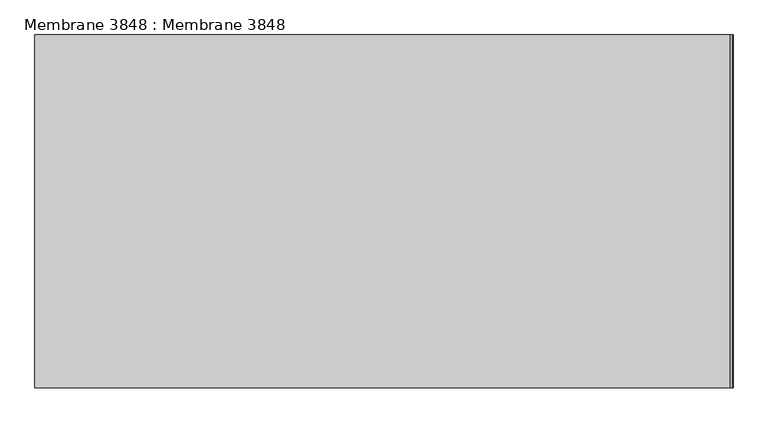
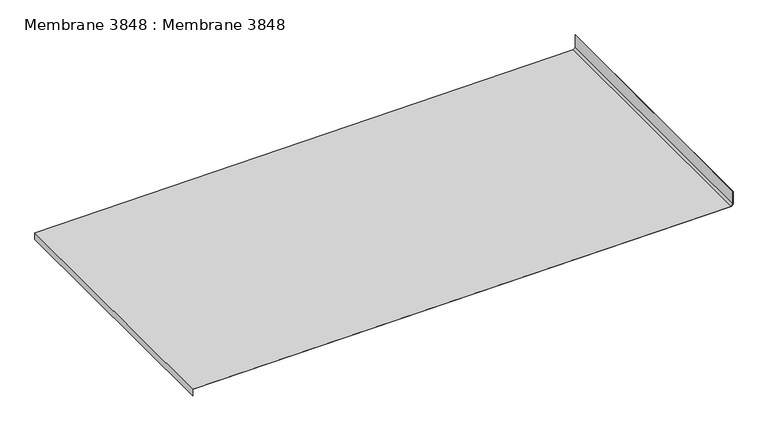
"""IFC4 building model written with IfcOpenShell, lengths in millimetres: proxy geometry, Membrane 3848 : Membrane 3848."""

from ifc_helpers import new_model, si_unit, frame, origin, place, context, project, spatial, polyline, outline, extrude, source, transform, mapped, element, save


def membrane_3848_membrane_3848_f9c4b706(model_context):
    return source(origin(), model_context, "Body", "SweptSolid", [
        extrude(outline(polyline([(36484.59375, -2108.1806641), (36471.7617187, -2122.0332031), (36433.25, -6061.9140625), (36381.4609375, -6061.9140625), (36381.4609375, -6059.9140625), (36431.2694541, -6059.9140625), (36469.7693673, -2121.2409559), (36483.7201769, -2106.1806641), (36581.6328125, -2106.1806641), (36581.6328125, -2108.1806641), (36484.59375, -2108.1806641)])), frame((0.0, -1052.8906574, 0.0), z_axis=(0.0, 1.0, 0.0), x_axis=(0.0, 0.0, 1.0)), (0.0, 0.0, 1.0), 2000.0),
    ])


if __name__ == "__main__":
    model = new_model("IFC4")
    model_context = context("Model", 3, world=origin())
    ifc_project = project(units=[si_unit("LENGTHUNIT", "METRE", prefix="MILLI")], contexts=[model_context])
    site = spatial("IfcSite", under=ifc_project)
    building = spatial("IfcBuilding", under=site)
    placement = place(None, origin())
    membrane_3848_membrane_3848_shape = membrane_3848_membrane_3848_f9c4b706(model_context)
    element("IfcBuildingElementProxy", 1, Name="Membrane 3848 : Membrane 3848", ObjectType="Membrane 3848 : Membrane 3848", at=placement, inside=building, context=model_context, shape_type="MappedRepresentation", body=[
        mapped(membrane_3848_membrane_3848_shape, transform((0.0, 0.0, 0.0), x_axis=(1.0, 0.0, 0.0), y_axis=(0.0, 1.0, 0.0), z_axis=(0.0, 0.0, 1.0))),
    ])
    save(model, "model.ifc")

# Revit data of these elements
# Type "Membrane 3848 : Membrane 3848"
#   NameOverride = "Membrane"
# Element 1 (IfcBuildingElementProxy, "Membrane 3848 : Membrane 3848")
#   Materials on its faces: "2 LAYERS NO. 30 ASTM D226 ASPHALT SATURATED ORGANIC FELT"
# Materials
#   "2 LAYERS NO. 30 ASTM D226 ASPHALT SATURATED ORGANIC FELT": class "Unassigned", colour RGB 46 171 0, transparency 0
